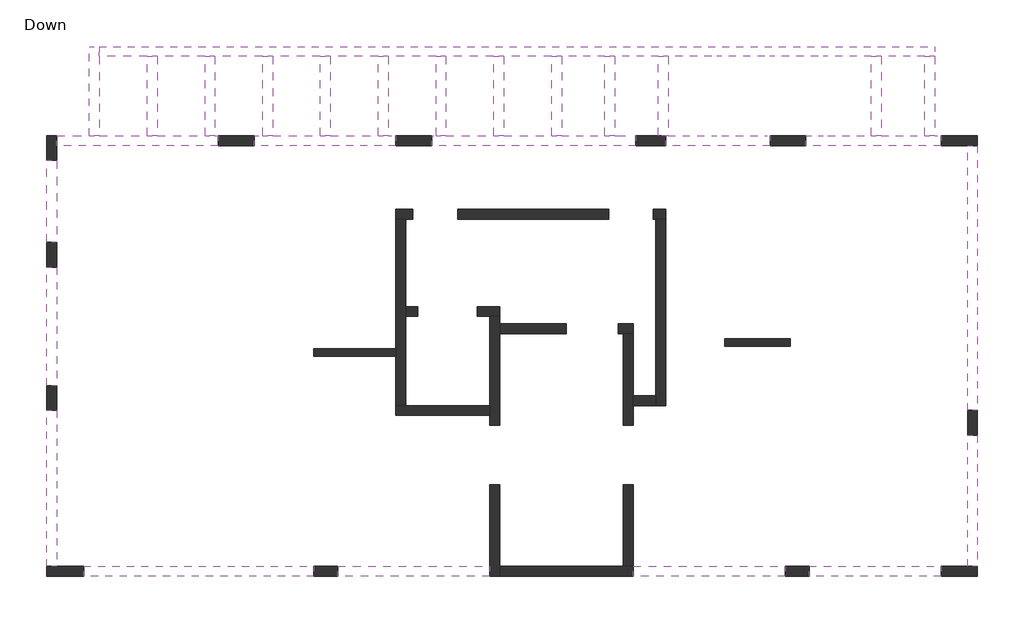
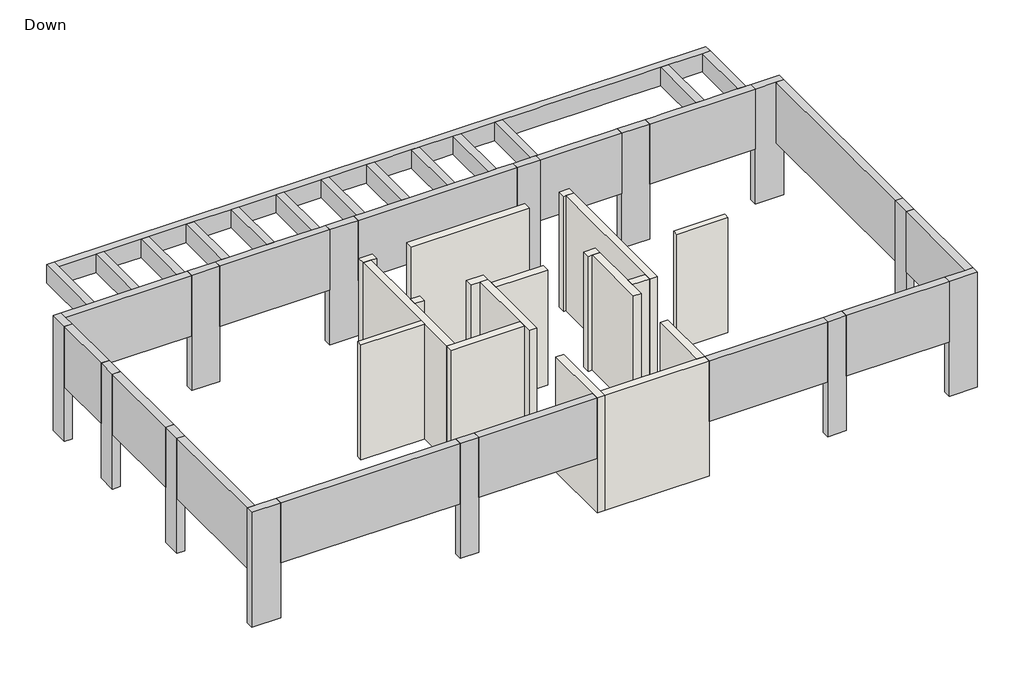
# One storey: 28 beams, 18 walls, 13 columns.
"""IFC4 building model written with IfcOpenShell, lengths in millimetres."""

from ifc_helpers import new_model, si_unit, frame, origin, origin_with_axes, place, context, project, spatial, polyline, outline, extrude, faceted_brep, element, save

model = new_model("IFC4")

# Units and contexts
model_context = context("Model", 3, world=origin())
ifc_project = project(units=[si_unit("LENGTHUNIT", "METRE", prefix="MILLI")], contexts=[model_context])

# Site, building, storey
site = spatial("IfcSite", under=ifc_project)
building = spatial("IfcBuilding", under=site)
storey = spatial("IfcBuildingStorey", under=building, Name="Down", Elevation=0.0)

# Beams
placement = place(None, origin())
element("IfcBeam", 1, ObjectType="Concrete Rectengular Beam : 20/165", at=placement, inside=storey, context=model_context, shape_type="SweptSolid", body=[
    extrude(outline(polyline([(-28799.0775982, 37234.7104697), (-28799.0775982, 37034.7104697), (-33449.2609999, 37034.7104697), (-33449.2609999, 37234.7104697), (-28799.0775982, 37234.7104697)])), frame((0.0, 0.0, 1500.0), z_axis=(0.0, 0.0, 1.0), x_axis=(1.0, 0.0, 0.0)), (0.0, 0.0, 1.0), 1650.0),
])
element("IfcBeam", 2, ObjectType="Concrete Rectengular Beam : 20/165", at=placement, inside=storey, context=model_context, shape_type="Brep", body=[
    faceted_brep([(-28319.0775982, 37234.7104697, 3150.0), (-28319.0775982, 37034.7104697, 3150.0), (-25248.1921114, 37034.7104697, 3150.0), (-25248.1921114, 37234.7104697, 3150.0), (-28319.0775982, 37034.7104697, 1500.0), (-25248.1921114, 37034.7104697, 1500.0), (-28319.0775982, 37234.7104697, 1500.0), (-25248.1921114, 37234.7104697, 1500.0), (-25248.1921114, 37234.7104697, 2950.0)], [[[0, 1, 2, 3]], [[1, 4, 5, 2]], [[4, 6, 7, 5]], [[6, 0, 3, 8, 7]], [[1, 0, 6, 4]], [[3, 2, 5, 7, 8]]]),
])
element("IfcBeam", 3, ObjectType="Concrete Rectengular Beam : 20/165", at=placement, inside=storey, context=model_context, shape_type="Brep", body=[
    faceted_brep([(-19279.0292046, 37034.7104697, 3150.0), (-19279.0292046, 37234.7104697, 3150.0), (-22348.1921114, 37234.7104697, 3150.0), (-22348.1921114, 37034.7104697, 3150.0), (-19279.0292046, 37034.7104697, 1500.0), (-22348.1921114, 37034.7104697, 1500.0), (-19279.0292046, 37234.7104697, 1500.0), (-22348.1921114, 37234.7104697, 1500.0), (-22348.1921114, 37234.7104697, 2950.0)], [[[0, 1, 2, 3]], [[4, 0, 3, 5]], [[6, 4, 5, 7]], [[1, 6, 7, 8, 2]], [[1, 0, 4, 6]], [[3, 2, 8, 7, 5]]]),
])
element("IfcBeam", 4, ObjectType="Concrete Rectengular Beam : 20/165", at=placement, inside=storey, context=model_context, shape_type="SweptSolid", body=[
    extrude(outline(polyline([(-16128.1921114, 37234.7104697), (-16128.1921114, 37034.7104697), (-18799.0292046, 37034.7104697), (-18799.0292046, 37234.7104697), (-16128.1921114, 37234.7104697)])), frame((0.0, 0.0, 1500.0), z_axis=(0.0, 0.0, 1.0), x_axis=(1.0, 0.0, 0.0)), (0.0, 0.0, 1.0), 1650.0),
])
element("IfcBeam", 5, ObjectType="Concrete Rectengular Beam : 20/165", at=placement, inside=storey, context=model_context, shape_type="Brep", body=[
    faceted_brep([(-15398.1921114, 39884.7076972, 3150.0), (-15598.1921114, 39884.7076972, 3150.0), (-15598.1921114, 37234.7104697, 3150.0), (-15398.1921114, 37234.7104697, 3150.0), (-15398.1921114, 39884.7076972, 1500.0), (-15398.1921114, 37234.7104697, 1500.0), (-15598.1921114, 39884.7076972, 1500.0), (-15598.1921114, 37234.7104697, 1500.0), (-15598.1921114, 37234.7104697, 2950.0)], [[[0, 1, 2, 3]], [[4, 0, 3, 5]], [[6, 4, 5, 7]], [[1, 6, 7, 8, 2]], [[1, 0, 4, 6]], [[3, 2, 8, 7, 5]]]),
])
element("IfcBeam", 6, ObjectType="Concrete Rectengular Beam : 20/165", at=placement, inside=storey, context=model_context, shape_type="Brep", body=[
    faceted_brep([(-15598.1921114, 40384.7076972, 3150.0), (-15398.1921114, 40384.7076972, 3150.0), (-15398.1921114, 45734.7104697, 3150.0), (-15598.1921114, 45734.7104697, 3150.0), (-15398.1921114, 40384.7076972, 1500.0), (-15398.1921114, 45734.7104697, 1500.0), (-15598.1921114, 40384.7076972, 1500.0), (-15598.1921114, 45734.7104697, 1500.0), (-15598.1921114, 45734.7104697, 2950.0)], [[[0, 1, 2, 3]], [[1, 4, 5, 2]], [[4, 6, 7, 5]], [[6, 0, 3, 8, 7]], [[1, 0, 6, 4]], [[3, 2, 5, 7, 8]]]),
])
element("IfcBeam", 7, ObjectType="Concrete Rectengular Beam : 20/165", at=placement, inside=storey, context=model_context, shape_type="Brep", body=[
    faceted_brep([(-16128.1921114, 45734.7104697, 3150.0), (-16128.1921114, 45934.7104697, 3150.0), (-16263.1921114, 45934.7104697, 3150.0), (-16463.1921114, 45934.7104697, 3150.0), (-17340.2921114, 45934.7104697, 3150.0), (-17540.2921114, 45934.7104697, 3150.0), (-18417.3921114, 45934.7104697, 3150.0), (-18617.3921114, 45934.7104697, 3150.0), (-18867.9882316, 45934.7104697, 3150.0), (-18867.9882316, 45734.7104697, 3150.0), (-16128.1921114, 45934.7104697, 1500.0), (-18867.9882316, 45934.7104697, 1500.0), (-16128.1921114, 45734.7104697, 1500.0), (-18867.9882316, 45734.7104697, 1500.0)], [[[0, 1, 2, 3, 4, 5, 6, 7, 8, 9]], [[1, 10, 11, 8, 7, 6, 5, 4, 3, 2]], [[10, 12, 13, 11]], [[12, 0, 9, 13]], [[1, 0, 12, 10]], [[9, 8, 11, 13]]]),
])
element("IfcBeam", 8, ObjectType="Concrete Rectengular Beam : 20/165", at=placement, inside=storey, context=model_context, shape_type="Brep", body=[
    faceted_brep([(-19587.9882316, 45734.7104697, 3150.0), (-19587.9882316, 45934.7104697, 3150.0), (-19694.4921114, 45934.7104697, 3150.0), (-20566.8921114, 45934.7104697, 3150.0), (-20766.8921114, 45934.7104697, 3150.0), (-21643.9921114, 45934.7104697, 3150.0), (-21697.8129925, 45934.7104697, 3150.0), (-21697.8129925, 45734.7104697, 3150.0), (-19587.9882316, 45934.7104697, 1500.0), (-21697.8129925, 45934.7104697, 1500.0), (-19587.9882316, 45734.7104697, 1500.0), (-21697.8129925, 45734.7104697, 1500.0)], [[[0, 1, 2, 3, 4, 5, 6, 7]], [[1, 8, 9, 6, 5, 4, 3, 2]], [[8, 10, 11, 9]], [[10, 0, 7, 11]], [[1, 0, 10, 8]], [[7, 6, 9, 11]]]),
])
element("IfcBeam", 9, ObjectType="Concrete Rectengular Beam : 20/165", at=placement, inside=storey, context=model_context, shape_type="Brep", body=[
    faceted_brep([(-26418.1921114, 45934.7104697, 3150.0), (-26418.1921114, 45734.7104697, 3150.0), (-22297.8129925, 45734.7104697, 3150.0), (-22297.8129925, 45934.7104697, 3150.0), (-22721.0921114, 45934.7104697, 3150.0), (-22921.0921114, 45934.7104697, 3150.0), (-23798.1921114, 45934.7104697, 3150.0), (-23998.1921114, 45934.7104697, 3150.0), (-24965.6921114, 45934.7104697, 3150.0), (-25165.6921114, 45934.7104697, 3150.0), (-26133.1921114, 45934.7104697, 3150.0), (-26333.1921114, 45934.7104697, 3150.0), (-26418.1921114, 45934.7104697, 1500.0), (-22297.8129925, 45934.7104697, 1500.0), (-26418.1921114, 45734.7104697, 1500.0), (-22297.8129925, 45734.7104697, 1500.0)], [[[0, 1, 2, 3, 4, 5, 6, 7, 8, 9, 10, 11]], [[12, 0, 11, 10, 9, 8, 7, 6, 5, 4, 3, 13]], [[14, 12, 13, 15]], [[1, 14, 15, 2]], [[1, 0, 12, 14]], [[3, 2, 15, 13]]]),
])
element("IfcBeam", 10, ObjectType="Concrete Rectengular Beam : 20/165", at=placement, inside=storey, context=model_context, shape_type="Brep", body=[
    faceted_brep([(-30003.1920714, 45934.7104697, 3150.0), (-30003.1920714, 45734.7104697, 3150.0), (-27148.1921114, 45734.7104697, 3150.0), (-27148.1921114, 45934.7104697, 3150.0), (-27300.6921114, 45934.7104697, 3150.0), (-27500.6921114, 45934.7104697, 3150.0), (-28468.1921114, 45934.7104697, 3150.0), (-28668.1921114, 45934.7104697, 3150.0), (-29630.6921114, 45934.7104697, 3150.0), (-29830.6921114, 45934.7104697, 3150.0), (-30003.1920714, 45934.7104697, 1500.0), (-27148.1921114, 45934.7104697, 1500.0), (-30003.1920714, 45734.7104697, 1500.0), (-27148.1921114, 45734.7104697, 1500.0)], [[[0, 1, 2, 3, 4, 5, 6, 7, 8, 9]], [[10, 0, 9, 8, 7, 6, 5, 4, 3, 11]], [[12, 10, 11, 13]], [[1, 12, 13, 2]], [[1, 0, 10, 12]], [[3, 2, 13, 11]]]),
])
element("IfcBeam", 11, ObjectType="Concrete Rectengular Beam : 20/165", at=placement, inside=storey, context=model_context, shape_type="Brep", body=[
    faceted_brep([(-33998.1921114, 45934.7104697, 3150.0), (-33998.1921114, 45734.7104697, 3150.0), (-30733.1920714, 45734.7104697, 3150.0), (-30733.1920714, 45934.7104697, 3150.0), (-30798.1921114, 45934.7104697, 3150.0), (-30998.1921114, 45934.7104697, 3150.0), (-31965.6921114, 45934.7104697, 3150.0), (-32165.6921114, 45934.7104697, 3150.0), (-33133.1921114, 45934.7104697, 3150.0), (-33333.1921114, 45934.7104697, 3150.0), (-33998.1921114, 45934.7104697, 1500.0), (-30733.1920714, 45934.7104697, 1500.0), (-33998.1921114, 45734.7104697, 1500.0), (-30733.1920714, 45734.7104697, 1500.0), (-33998.1921114, 45734.7104697, 2950.0)], [[[0, 1, 2, 3, 4, 5, 6, 7, 8, 9]], [[10, 0, 9, 8, 7, 6, 5, 4, 3, 11]], [[12, 10, 11, 13]], [[1, 14, 12, 13, 2]], [[1, 0, 10, 12, 14]], [[3, 2, 13, 11]]]),
])
element("IfcBeam", 12, ObjectType="Concrete Rectengular Beam : 20/165", at=placement, inside=storey, context=model_context, shape_type="SweptSolid", body=[
    extrude(outline(polyline([(-34198.1921114, 45434.7104697), (-33998.1921114, 45434.7104697), (-33998.1921114, 43778.8121651), (-34198.1921114, 43778.8121651), (-34198.1921114, 45434.7104697)])), frame((0.0, 0.0, 1500.0), z_axis=(0.0, 0.0, 1.0), x_axis=(1.0, 0.0, 0.0)), (0.0, 0.0, 1.0), 1650.0),
])
element("IfcBeam", 13, ObjectType="Concrete Rectengular Beam : 20/165", at=placement, inside=storey, context=model_context, shape_type="SweptSolid", body=[
    extrude(outline(polyline([(-34198.1921114, 43278.8121651), (-33998.1921114, 43278.8121651), (-33998.1921114, 40884.7121321), (-34198.1921114, 40884.7121321), (-34198.1921114, 43278.8121651)])), frame((0.0, 0.0, 1500.0), z_axis=(0.0, 0.0, 1.0), x_axis=(1.0, 0.0, 0.0)), (0.0, 0.0, 1.0), 1650.0),
])
element("IfcBeam", 14, ObjectType="Concrete Rectengular Beam : 20/165", at=placement, inside=storey, context=model_context, shape_type="Brep", body=[
    faceted_brep([(-33998.1921114, 40384.7121321, 3150.0), (-34198.1921114, 40384.7121321, 3150.0), (-34198.1921114, 37234.7104697, 3150.0), (-33998.1921114, 37234.7104697, 3150.0), (-34198.1921114, 40384.7121321, 1500.0), (-34198.1921114, 37234.7104697, 1500.0), (-33998.1921114, 40384.7121321, 1500.0), (-33998.1921114, 37234.7104697, 1500.0), (-33998.1921114, 37234.7104697, 2950.0)], [[[0, 1, 2, 3]], [[1, 4, 5, 2]], [[4, 6, 7, 5]], [[6, 0, 3, 8, 7]], [[1, 0, 6, 4]], [[3, 2, 5, 7, 8]]]),
])
element("IfcBeam", 15, ObjectType="Concrete Rectengular Beam : 20/50", at=placement, inside=storey, context=model_context, shape_type="Brep", body=[
    faceted_brep([(-33133.1921114, 47734.7104697, 3150.0), (-33333.1921114, 47734.7104697, 3150.0), (-33333.1921114, 45934.7104697, 3150.0), (-33133.1921114, 45934.7104697, 3150.0), (-33133.1921114, 47534.7104697, 3150.0), (-33133.1921114, 47734.7104697, 2650.0), (-33133.1921114, 45934.7104697, 2650.0), (-33133.1921114, 47534.7104697, 2650.0), (-33333.1921114, 47734.7104697, 2650.0), (-33333.1921114, 45934.7104697, 2650.0)], [[[0, 1, 2, 3, 4]], [[5, 0, 4, 3, 6, 7]], [[8, 5, 7, 6, 9]], [[1, 8, 9, 2]], [[3, 2, 9, 6]], [[1, 0, 5, 8]]]),
])
element("IfcBeam", 16, ObjectType="Concrete Rectengular Beam : 20/50", at=placement, inside=storey, context=model_context, shape_type="Brep", body=[
    faceted_brep([(-16263.1921114, 47534.7104697, 3150.0), (-16263.1921114, 47734.7104697, 3150.0), (-33133.1921114, 47734.7104697, 3150.0), (-33133.1921114, 47534.7104697, 3150.0), (-32165.6921114, 47534.7104697, 3150.0), (-31965.6921114, 47534.7104697, 3150.0), (-30998.1921114, 47534.7104697, 3150.0), (-30798.1921114, 47534.7104697, 3150.0), (-29830.6921114, 47534.7104697, 3150.0), (-29630.6921114, 47534.7104697, 3150.0), (-28668.1921114, 47534.7104697, 3150.0), (-28468.1921114, 47534.7104697, 3150.0), (-27500.6921114, 47534.7104697, 3150.0), (-27300.6921114, 47534.7104697, 3150.0), (-26333.1921114, 47534.7104697, 3150.0), (-26133.1921114, 47534.7104697, 3150.0), (-25165.6921114, 47534.7104697, 3150.0), (-24965.6921114, 47534.7104697, 3150.0), (-23998.1921114, 47534.7104697, 3150.0), (-23798.1921114, 47534.7104697, 3150.0), (-22921.0921114, 47534.7104697, 3150.0), (-22721.0921114, 47534.7104697, 3150.0), (-21843.9921114, 47534.7104697, 3150.0), (-21643.9921114, 47534.7104697, 3150.0), (-20766.8921114, 47534.7104697, 3150.0), (-20566.8921114, 47534.7104697, 3150.0), (-19694.4921114, 47534.7104697, 3150.0), (-19494.4921114, 47534.7104697, 3150.0), (-18617.3921114, 47534.7104697, 3150.0), (-18417.3921114, 47534.7104697, 3150.0), (-17540.2921114, 47534.7104697, 3150.0), (-17340.2921114, 47534.7104697, 3150.0), (-16463.1921114, 47534.7104697, 3150.0), (-16263.1921114, 47534.7104697, 2650.0), (-33133.1921114, 47534.7104697, 2650.0), (-32165.6921114, 47534.7104697, 2650.0), (-31965.6921114, 47534.7104697, 2650.0), (-30998.1921114, 47534.7104697, 2650.0), (-30798.1921114, 47534.7104697, 2650.0), (-29830.6921114, 47534.7104697, 2650.0), (-29630.6921114, 47534.7104697, 2650.0), (-28668.1921114, 47534.7104697, 2650.0), (-28468.1921114, 47534.7104697, 2650.0), (-27500.6921114, 47534.7104697, 2650.0), (-27300.6921114, 47534.7104697, 2650.0), (-26333.1921114, 47534.7104697, 2650.0), (-26133.1921114, 47534.7104697, 2650.0), (-25165.6921114, 47534.7104697, 2650.0), (-24965.6921114, 47534.7104697, 2650.0), (-23998.1921114, 47534.7104697, 2650.0), (-23798.1921114, 47534.7104697, 2650.0), (-22921.0921114, 47534.7104697, 2650.0), (-22721.0921114, 47534.7104697, 2650.0), (-21843.9921114, 47534.7104697, 2650.0), (-21643.9921114, 47534.7104697, 2650.0), (-20766.8921114, 47534.7104697, 2650.0), (-20566.8921114, 47534.7104697, 2650.0), (-19694.4921114, 47534.7104697, 2650.0), (-19494.4921114, 47534.7104697, 2650.0), (-18617.3921114, 47534.7104697, 2650.0), (-18417.3921114, 47534.7104697, 2650.0), (-17540.2921114, 47534.7104697, 2650.0), (-17340.2921114, 47534.7104697, 2650.0), (-16463.1921114, 47534.7104697, 2650.0), (-16263.1921114, 47734.7104697, 2650.0), (-33133.1921114, 47734.7104697, 2650.0)], [[[0, 1, 2, 3, 4, 5, 6, 7, 8, 9, 10, 11, 12, 13, 14, 15, 16, 17, 18, 19, 20, 21, 22, 23, 24, 25, 26, 27, 28, 29, 30, 31, 32]], [[33, 0, 32, 31, 30, 29, 28, 27, 26, 25, 24, 23, 22, 21, 20, 19, 18, 17, 16, 15, 14, 13, 12, 11, 10, 9, 8, 7, 6, 5, 4, 3, 34, 35, 36, 37, 38, 39, 40, 41, 42, 43, 44, 45, 46, 47, 48, 49, 50, 51, 52, 53, 54, 55, 56, 57, 58, 59, 60, 61, 62, 63]], [[64, 33, 63, 62, 61, 60, 59, 58, 57, 56, 55, 54, 53, 52, 51, 50, 49, 48, 47, 46, 45, 44, 43, 42, 41, 40, 39, 38, 37, 36, 35, 34, 65]], [[1, 64, 65, 2]], [[3, 2, 65, 34]], [[1, 0, 33, 64]]]),
])
element("IfcBeam", 17, ObjectType="Concrete Rectengular Beam : 20/50", at=placement, inside=storey, context=model_context, shape_type="SweptSolid", body=[
    extrude(outline(polyline([(-16463.1921114, 47534.7104697), (-16263.1921114, 47534.7104697), (-16263.1921114, 45934.7104697), (-16463.1921114, 45934.7104697), (-16463.1921114, 47534.7104697)])), frame((0.0, 0.0, 2650.0), z_axis=(0.0, 0.0, 1.0), x_axis=(1.0, 0.0, 0.0)), (0.0, 0.0, 1.0), 500.0),
])
element("IfcBeam", 18, ObjectType="Concrete Rectengular Beam : 20/50", at=placement, inside=storey, context=model_context, shape_type="SweptSolid", body=[
    extrude(outline(polyline([(-17540.2921114, 47534.7104697), (-17340.2921114, 47534.7104697), (-17340.2921114, 45934.7104697), (-17540.2921114, 45934.7104697), (-17540.2921114, 47534.7104697)])), frame((0.0, 0.0, 2650.0), z_axis=(0.0, 0.0, 1.0), x_axis=(1.0, 0.0, 0.0)), (0.0, 0.0, 1.0), 500.0),
])
element("IfcBeam", 19, ObjectType="Concrete Rectengular Beam : 20/50", at=placement, inside=storey, context=model_context, shape_type="Brep", body=[
    faceted_brep([(-21843.9921114, 45934.7104697, 3150.0), (-21697.8129925, 45934.7104697, 3150.0), (-21643.9921114, 45934.7104697, 3150.0), (-21643.9921114, 47534.7104697, 3150.0), (-21843.9921114, 47534.7104697, 3150.0), (-21843.9921114, 45934.7104697, 2650.0), (-21843.9921114, 47534.7104697, 2650.0), (-21643.9921114, 45934.7104697, 2650.0), (-21643.9921114, 47534.7104697, 2650.0)], [[[0, 1, 2, 3, 4]], [[5, 0, 4, 6]], [[7, 5, 6, 8]], [[2, 7, 8, 3]], [[2, 1, 0, 5, 7]], [[4, 3, 8, 6]]]),
])
element("IfcBeam", 20, ObjectType="Concrete Rectengular Beam : 20/50", at=placement, inside=storey, context=model_context, shape_type="SweptSolid", body=[
    extrude(outline(polyline([(-22921.0921114, 47534.7104697), (-22721.0921114, 47534.7104697), (-22721.0921114, 45934.7104697), (-22921.0921114, 45934.7104697), (-22921.0921114, 47534.7104697)])), frame((0.0, 0.0, 2650.0), z_axis=(0.0, 0.0, 1.0), x_axis=(1.0, 0.0, 0.0)), (0.0, 0.0, 1.0), 500.0),
])
element("IfcBeam", 21, ObjectType="Concrete Rectengular Beam : 20/50", at=placement, inside=storey, context=model_context, shape_type="SweptSolid", body=[
    extrude(outline(polyline([(-23798.1921114, 45934.7104697), (-23998.1921114, 45934.7104697), (-23998.1921114, 47534.7104697), (-23798.1921114, 47534.7104697), (-23798.1921114, 45934.7104697)])), frame((0.0, 0.0, 2650.0), z_axis=(0.0, 0.0, 1.0), x_axis=(1.0, 0.0, 0.0)), (0.0, 0.0, 1.0), 500.0),
])
element("IfcBeam", 22, ObjectType="Concrete Rectengular Beam : 20/50", at=placement, inside=storey, context=model_context, shape_type="SweptSolid", body=[
    extrude(outline(polyline([(-24965.6921114, 45934.7104697), (-25165.6921114, 45934.7104697), (-25165.6921114, 47534.7104697), (-24965.6921114, 47534.7104697), (-24965.6921114, 45934.7104697)])), frame((0.0, 0.0, 2650.0), z_axis=(0.0, 0.0, 1.0), x_axis=(1.0, 0.0, 0.0)), (0.0, 0.0, 1.0), 500.0),
])
element("IfcBeam", 23, ObjectType="Concrete Rectengular Beam : 20/50", at=placement, inside=storey, context=model_context, shape_type="SweptSolid", body=[
    extrude(outline(polyline([(-26133.1921114, 45934.7104697), (-26333.1921114, 45934.7104697), (-26333.1921114, 47534.7104697), (-26133.1921114, 47534.7104697), (-26133.1921114, 45934.7104697)])), frame((0.0, 0.0, 2650.0), z_axis=(0.0, 0.0, 1.0), x_axis=(1.0, 0.0, 0.0)), (0.0, 0.0, 1.0), 500.0),
])
element("IfcBeam", 24, ObjectType="Concrete Rectengular Beam : 20/50", at=placement, inside=storey, context=model_context, shape_type="SweptSolid", body=[
    extrude(outline(polyline([(-27500.6921114, 47534.7104697), (-27300.6921114, 47534.7104697), (-27300.6921114, 45934.7104697), (-27500.6921114, 45934.7104697), (-27500.6921114, 47534.7104697)])), frame((0.0, 0.0, 2650.0), z_axis=(0.0, 0.0, 1.0), x_axis=(1.0, 0.0, 0.0)), (0.0, 0.0, 1.0), 500.0),
])
element("IfcBeam", 25, ObjectType="Concrete Rectengular Beam : 20/50", at=placement, inside=storey, context=model_context, shape_type="SweptSolid", body=[
    extrude(outline(polyline([(-28468.1921114, 45934.7104697), (-28668.1921114, 45934.7104697), (-28668.1921114, 47534.7104697), (-28468.1921114, 47534.7104697), (-28468.1921114, 45934.7104697)])), frame((0.0, 0.0, 2650.0), z_axis=(0.0, 0.0, 1.0), x_axis=(1.0, 0.0, 0.0)), (0.0, 0.0, 1.0), 500.0),
])
element("IfcBeam", 26, ObjectType="Concrete Rectengular Beam : 20/50", at=placement, inside=storey, context=model_context, shape_type="SweptSolid", body=[
    extrude(outline(polyline([(-29630.6921114, 45934.7104697), (-29830.6921114, 45934.7104697), (-29830.6921114, 47534.7104697), (-29630.6921114, 47534.7104697), (-29630.6921114, 45934.7104697)])), frame((0.0, 0.0, 2650.0), z_axis=(0.0, 0.0, 1.0), x_axis=(1.0, 0.0, 0.0)), (0.0, 0.0, 1.0), 500.0),
])
element("IfcBeam", 27, ObjectType="Concrete Rectengular Beam : 20/50", at=placement, inside=storey, context=model_context, shape_type="SweptSolid", body=[
    extrude(outline(polyline([(-30798.1921114, 45934.7104697), (-30998.1921114, 45934.7104697), (-30998.1921114, 47534.7104697), (-30798.1921114, 47534.7104697), (-30798.1921114, 45934.7104697)])), frame((0.0, 0.0, 2650.0), z_axis=(0.0, 0.0, 1.0), x_axis=(1.0, 0.0, 0.0)), (0.0, 0.0, 1.0), 500.0),
])
element("IfcBeam", 28, ObjectType="Concrete Rectengular Beam : 20/50", at=placement, inside=storey, context=model_context, shape_type="SweptSolid", body=[
    extrude(outline(polyline([(-31965.6921114, 45934.7104697), (-32165.6921114, 45934.7104697), (-32165.6921114, 47534.7104697), (-31965.6921114, 47534.7104697), (-31965.6921114, 45934.7104697)])), frame((0.0, 0.0, 2650.0), z_axis=(0.0, 0.0, 1.0), x_axis=(1.0, 0.0, 0.0)), (0.0, 0.0, 1.0), 500.0),
])

# Columns
element("IfcColumn", 29, ObjectType="Concrete Rectengular Column : 20/48", at=placement, inside=storey, context=model_context, shape_type="SweptSolid", body=[
    extrude(outline(polyline([(-28799.0775982, 37234.7104697), (-28319.0775982, 37234.7104697), (-28319.0775982, 37034.7104697), (-28799.0775982, 37034.7104697), (-28799.0775982, 37234.7104697)])), origin_with_axes(), (0.0, 0.0, 1.0), 3150.0),
])
element("IfcColumn", 30, ObjectType="Concrete Rectengular Column : 20/48", at=placement, inside=storey, context=model_context, shape_type="SweptSolid", body=[
    extrude(outline(polyline([(-19279.0292046, 37234.7104697), (-18799.0292046, 37234.7104697), (-18799.0292046, 37034.7104697), (-19279.0292046, 37034.7104697), (-19279.0292046, 37234.7104697)])), origin_with_axes(), (0.0, 0.0, 1.0), 3150.0),
])
element("IfcColumn", 31, ObjectType="Concrete Rectengular Column : 20/50", at=placement, inside=storey, context=model_context, shape_type="Brep", body=[
    faceted_brep([(-33998.1921114, 45934.7104697, 0.0), (-33998.1921114, 45434.7104697, 0.0), (-34198.1921114, 45434.7104697, 0.0), (-34198.1921114, 45934.7104697, 0.0), (-33998.1921114, 45934.7104697, 3150.0), (-33998.1921114, 45734.7104697, 3150.0), (-33998.1921114, 45434.7104697, 3150.0), (-34198.1921114, 45434.7104697, 3150.0), (-34198.1921114, 45934.7104697, 3150.0)], [[[0, 1, 2, 3]], [[4, 5, 6, 1, 0]], [[6, 7, 2, 1]], [[7, 8, 3, 2]], [[8, 4, 0, 3]], [[4, 8, 7, 6, 5]]]),
])
element("IfcColumn", 32, ObjectType="Concrete Rectengular Column : 20/50", at=placement, inside=storey, context=model_context, shape_type="SweptSolid", body=[
    extrude(outline(polyline([(-33998.1921114, 43778.8121651), (-33998.1921114, 43278.8121651), (-34198.1921114, 43278.8121651), (-34198.1921114, 43778.8121651), (-33998.1921114, 43778.8121651)])), origin_with_axes(), (0.0, 0.0, 1.0), 3150.0),
])
element("IfcColumn", 33, ObjectType="Concrete Rectengular Column : 20/50", at=placement, inside=storey, context=model_context, shape_type="SweptSolid", body=[
    extrude(outline(polyline([(-33998.1921114, 40884.7121321), (-33998.1921114, 40384.7121321), (-34198.1921114, 40384.7121321), (-34198.1921114, 40884.7121321), (-33998.1921114, 40884.7121321)])), origin_with_axes(), (0.0, 0.0, 1.0), 3150.0),
])
element("IfcColumn", 34, ObjectType="Concrete Rectengular Column : 20/50", at=placement, inside=storey, context=model_context, shape_type="SweptSolid", body=[
    extrude(outline(polyline([(-15398.1921114, 40384.7076972), (-15398.1921114, 39884.7076972), (-15598.1921114, 39884.7076972), (-15598.1921114, 40384.7076972), (-15398.1921114, 40384.7076972)])), origin_with_axes(), (0.0, 0.0, 1.0), 3150.0),
])
element("IfcColumn", 35, ObjectType="Concrete Rectengular Column : 20/60", at=placement, inside=storey, context=model_context, shape_type="Brep", body=[
    faceted_brep([(-22297.8129925, 45934.7104697, 0.0), (-21697.8129925, 45934.7104697, 0.0), (-21697.8129925, 45734.7104697, 0.0), (-22297.8129925, 45734.7104697, 0.0), (-22297.8129925, 45934.7104697, 3150.0), (-21697.8129925, 45934.7104697, 3150.0), (-22297.8129925, 45934.7104697, 1500.0), (-21697.8129925, 45734.7104697, 3150.0), (-21698.192111, 45734.7104697, 3150.0), (-22297.8129925, 45734.7104697, 3150.0), (-22297.8129925, 45734.7104697, 1500.0)], [[[0, 1, 2, 3]], [[4, 5, 1, 0, 6]], [[5, 7, 2, 1]], [[7, 8, 9, 10, 3, 2]], [[9, 4, 6, 0, 3, 10]], [[4, 9, 8, 7, 5]]]),
])
element("IfcColumn", 36, ObjectType="Concrete Rectengular Column : 20/72", at=placement, inside=storey, context=model_context, shape_type="SweptSolid", body=[
    extrude(outline(polyline([(-19587.9882316, 45934.7104697), (-18867.9882316, 45934.7104697), (-18867.9882316, 45734.7104697), (-19587.9882316, 45734.7104697), (-19587.9882316, 45934.7104697)])), origin_with_axes(), (0.0, 0.0, 1.0), 3150.0),
])
element("IfcColumn", 37, ObjectType="Concrete Rectengular Column : 20/73", at=placement, inside=storey, context=model_context, shape_type="Brep", body=[
    faceted_brep([(-16128.1921114, 37234.7104697, 0.0), (-15398.1921114, 37234.7104697, 0.0), (-15398.1921114, 37034.7104697, 0.0), (-16128.1921114, 37034.7104697, 0.0), (-16128.1921114, 37234.7104697, 3150.0), (-15598.1921114, 37234.7104697, 3150.0), (-15398.1921114, 37234.7104697, 3150.0), (-15398.1921114, 37034.7104697, 3150.0), (-16128.1921114, 37034.7104697, 3150.0)], [[[0, 1, 2, 3]], [[4, 5, 6, 1, 0]], [[6, 7, 2, 1]], [[7, 8, 3, 2]], [[8, 4, 0, 3]], [[4, 8, 7, 6, 5]]]),
])
element("IfcColumn", 38, ObjectType="Concrete Rectengular Column : 20/73", at=placement, inside=storey, context=model_context, shape_type="Brep", body=[
    faceted_brep([(-16128.1921114, 45934.7104697, 0.0), (-15398.1921114, 45934.7104697, 0.0), (-15398.1921114, 45734.7104697, 0.0), (-16128.1921114, 45734.7104697, 0.0), (-16128.1921114, 45934.7104697, 3150.0), (-15398.1921114, 45934.7104697, 3150.0), (-15398.1921114, 45734.7104697, 3150.0), (-15598.1921114, 45734.7104697, 3150.0), (-16128.1921114, 45734.7104697, 3150.0)], [[[0, 1, 2, 3]], [[4, 5, 1, 0]], [[5, 6, 2, 1]], [[6, 7, 8, 3, 2]], [[8, 4, 0, 3]], [[4, 8, 7, 6, 5]]]),
])
element("IfcColumn", 39, ObjectType="Concrete Rectengular Column : 20/73", at=placement, inside=storey, context=model_context, shape_type="SweptSolid", body=[
    extrude(outline(polyline([(-30733.1920714, 45934.7104697), (-30003.1920714, 45934.7104697), (-30003.1920714, 45734.7104697), (-30733.1920714, 45734.7104697), (-30733.1920714, 45934.7104697)])), origin_with_axes(), (0.0, 0.0, 1.0), 3150.0),
])
element("IfcColumn", 40, ObjectType="Concrete Rectengular Column : 20/73", at=placement, inside=storey, context=model_context, shape_type="SweptSolid", body=[
    extrude(outline(polyline([(-27148.1921114, 45934.7104697), (-26418.1921114, 45934.7104697), (-26418.1921114, 45734.7104697), (-27148.1921114, 45734.7104697), (-27148.1921114, 45934.7104697)])), origin_with_axes(), (0.0, 0.0, 1.0), 3150.0),
])
element("IfcColumn", 41, ObjectType="Concrete Rectengular Column : 20/75", at=placement, inside=storey, context=model_context, shape_type="Brep", body=[
    faceted_brep([(-34199.2609999, 37234.7104697, 0.0), (-33449.2609999, 37234.7104697, 0.0), (-33449.2609999, 37034.7104697, 0.0), (-34199.2609999, 37034.7104697, 0.0), (-34199.2609999, 37234.7104697, 3150.0), (-33998.1921114, 37234.7104697, 3150.0), (-33449.2609999, 37234.7104697, 3150.0), (-33449.2609999, 37034.7104697, 3150.0), (-34199.2609999, 37034.7104697, 3150.0)], [[[0, 1, 2, 3]], [[4, 5, 6, 1, 0]], [[6, 7, 2, 1]], [[7, 8, 3, 2]], [[8, 4, 0, 3]], [[4, 8, 7, 6, 5]]]),
])

# Walls
element("IfcWall", 42, ObjectType="15", at=placement, inside=storey, context=model_context, shape_type="Brep", body=[
    faceted_brep([(-28798.1921114, 41484.7104697, 0.0), (-27148.1921114, 41484.7104697, 0.0), (-27148.1921114, 41484.7104697, 2950.0), (-27148.1921114, 41484.7104697, 3150.0), (-28798.1921114, 41484.7104697, 3150.0), (-28798.1921114, 41484.7104697, 2950.0), (-28798.1921114, 41634.7104697, 0.0), (-28798.1921114, 41634.7104697, 2950.0), (-28798.1921114, 41634.7104697, 3150.0), (-27148.1921114, 41634.7104697, 3150.0), (-27148.1921114, 41634.7104697, 2950.0), (-27148.1921114, 41634.7104697, 0.0)], [[[0, 1, 2, 3, 4, 5]], [[6, 7, 8, 9, 10, 11]], [[1, 0, 6, 11]], [[4, 3, 9, 8]], [[0, 5, 4, 8, 7, 6]], [[3, 2, 1, 11, 10, 9]]]),
])
element("IfcWall", 43, ObjectType="15", at=placement, inside=storey, context=model_context, shape_type="Brep", body=[
    faceted_brep([(-19178.1921114, 41834.7104349, 0.0), (-20498.1921114, 41834.7104349, 0.0), (-20498.1921114, 41834.7104349, 2950.0), (-20498.1921114, 41834.7104349, 3150.0), (-19178.1921114, 41834.7104349, 3150.0), (-19178.1921114, 41834.7104349, 2950.0), (-19178.1921114, 41684.7104349, 0.0), (-19178.1921114, 41684.7104349, 2950.0), (-19178.1921114, 41684.7104349, 3150.0), (-20498.1921114, 41684.7104349, 3150.0), (-20498.1921114, 41684.7104349, 2950.0), (-20498.1921114, 41684.7104349, 0.0)], [[[0, 1, 2, 3, 4, 5]], [[6, 7, 8, 9, 10, 11]], [[1, 0, 6, 11]], [[3, 2, 1, 11, 10, 9]], [[4, 3, 9, 8]], [[0, 5, 4, 8, 7, 6]]]),
])
element("IfcWall", 44, ObjectType="20", at=placement, inside=storey, context=model_context, shape_type="Brep", body=[
    faceted_brep([(-25248.1921114, 38884.7104697, 0.0), (-25248.1921114, 37034.7104697, 0.0), (-25248.1921114, 37034.7104697, 3150.0), (-25248.1921114, 37234.7104697, 3150.0), (-25248.1921114, 38884.7104697, 3150.0), (-25248.1921114, 38884.7104697, 2950.0), (-25048.1921114, 38884.7104697, 0.0), (-25048.1921114, 38884.7104697, 2950.0), (-25048.1921114, 38884.7104697, 3150.0), (-25048.1921114, 37234.7104697, 3150.0), (-25048.1921114, 37034.7104697, 3150.0), (-25048.1921114, 37034.7104697, 0.0), (-25048.1921114, 37234.7104697, 0.0)], [[[0, 1, 2, 3, 4, 5]], [[6, 7, 8, 9, 10, 11, 12]], [[1, 0, 6, 12, 11]], [[4, 3, 2, 10, 9, 8]], [[0, 5, 4, 8, 7, 6]], [[2, 1, 11, 10]]]),
])
element("IfcWall", 45, ObjectType="20", at=placement, inside=storey, context=model_context, shape_type="Brep", body=[
    faceted_brep([(-25048.1921114, 37034.7104697, 0.0), (-22348.1921114, 37034.7104697, 0.0), (-22348.1921114, 37034.7104697, 1500.0), (-22348.1921114, 37034.7104697, 3150.0), (-25048.1921114, 37034.7104697, 3150.0), (-25048.1921114, 37234.7104697, 0.0), (-25048.1921114, 37234.7104697, 3150.0), (-22548.1921114, 37234.7104697, 3150.0), (-22348.1921114, 37234.7104697, 3150.0), (-22348.1921114, 37234.7104697, 1500.0), (-22348.1921114, 37234.7104697, 0.0), (-22548.1921114, 37234.7104697, 0.0)], [[[0, 1, 2, 3, 4]], [[5, 6, 7, 8, 9, 10, 11]], [[1, 0, 5, 11, 10]], [[4, 3, 8, 7, 6]], [[0, 4, 6, 5]], [[3, 2, 1, 10, 9, 8]]]),
])
element("IfcWall", 46, ObjectType="20", at=placement, inside=storey, context=model_context, shape_type="Brep", body=[
    faceted_brep([(-22348.1921114, 37234.7104697, 0.0), (-22348.1921114, 38884.7104697, 0.0), (-22348.1921114, 38884.7104697, 2950.0), (-22348.1921114, 38884.7104697, 3150.0), (-22348.1921114, 37234.7104697, 3150.0), (-22348.1921114, 37234.7104697, 2950.0), (-22548.1921114, 37234.7104697, 0.0), (-22548.1921114, 37234.7104697, 3150.0), (-22548.1921114, 38884.7104697, 3150.0), (-22548.1921114, 38884.7104697, 2950.0), (-22548.1921114, 38884.7104697, 0.0)], [[[0, 1, 2, 3, 4, 5]], [[6, 7, 8, 9, 10]], [[1, 0, 6, 10]], [[3, 2, 1, 10, 9, 8]], [[4, 3, 8, 7]], [[0, 5, 4, 7, 6]]]),
])
element("IfcWall", 47, ObjectType="20", at=placement, inside=storey, context=model_context, shape_type="Brep", body=[
    faceted_brep([(-22348.1921114, 40084.7104697, 0.0), (-22348.1921114, 40484.7104697, 0.0), (-22348.1921114, 40684.7104697, 0.0), (-22348.1921114, 41934.7104698, 0.0), (-22348.1921114, 41934.7104698, 3150.0), (-22348.1921114, 40684.7104697, 3150.0), (-22348.1921114, 40484.7104697, 3150.0), (-22348.1921114, 40084.7104697, 3150.0), (-22348.1921114, 40084.7104697, 2950.0), (-22548.1921114, 40084.7104697, 0.0), (-22548.1921114, 40084.7104697, 2950.0), (-22548.1921114, 40084.7104697, 3150.0), (-22548.1921114, 41934.7104698, 3150.0), (-22548.1921114, 41934.7104698, 0.0)], [[[0, 1, 2, 3, 4, 5, 6, 7, 8]], [[9, 10, 11, 12, 13]], [[3, 2, 1, 0, 9, 13]], [[7, 6, 5, 4, 12, 11]], [[0, 8, 7, 11, 10, 9]], [[4, 3, 13, 12]]]),
])
element("IfcWall", 48, ObjectType="20", at=placement, inside=storey, context=model_context, shape_type="Brep", body=[
    faceted_brep([(-22348.1921114, 42134.7104698, 0.0), (-22648.1921114, 42134.7104698, 0.0), (-22648.1921114, 42134.7104698, 2950.0), (-22648.1921114, 42134.7104698, 3150.0), (-22348.1921114, 42134.7104698, 3150.0), (-22348.1921114, 42134.7104698, 2950.0), (-22348.1921114, 41934.7104698, 0.0), (-22348.1921114, 41934.7104698, 3150.0), (-22548.1921114, 41934.7104698, 3150.0), (-22648.1921114, 41934.7104698, 3150.0), (-22648.1921114, 41934.7104698, 2950.0), (-22648.1921114, 41934.7104698, 0.0), (-22548.1921114, 41934.7104698, 0.0)], [[[0, 1, 2, 3, 4, 5]], [[6, 7, 8, 9, 10, 11, 12]], [[1, 0, 6, 12, 11]], [[3, 2, 1, 11, 10, 9]], [[4, 3, 9, 8, 7]], [[0, 5, 4, 7, 6]]]),
])
element("IfcWall", 49, ObjectType="20", at=placement, inside=storey, context=model_context, shape_type="Brep", body=[
    faceted_brep([(-23698.1921114, 42134.7104697, 0.0), (-25048.1921114, 42134.7104697, 0.0), (-25048.1921114, 42134.7104697, 2950.0), (-25048.1921114, 42134.7104697, 3150.0), (-23698.1921114, 42134.7104697, 3150.0), (-23698.1921114, 42134.7104697, 2950.0), (-23698.1921114, 41934.7104697, 0.0), (-23698.1921114, 41934.7104697, 2950.0), (-23698.1921114, 41934.7104697, 3150.0), (-25048.1921114, 41934.7104697, 3150.0), (-25048.1921114, 41934.7104697, 0.0)], [[[0, 1, 2, 3, 4, 5]], [[6, 7, 8, 9, 10]], [[1, 0, 6, 10]], [[4, 3, 9, 8]], [[0, 5, 4, 8, 7, 6]], [[3, 2, 1, 10, 9]]]),
])
element("IfcWall", 50, ObjectType="20", at=placement, inside=storey, context=model_context, shape_type="Brep", body=[
    faceted_brep([(-25248.1921114, 42284.7104696, 0.0), (-25248.1921114, 40484.7104697, 0.0), (-25248.1921114, 40284.7104697, 0.0), (-25248.1921114, 40084.7104697, 0.0), (-25248.1921114, 40084.7104697, 2950.0), (-25248.1921114, 40084.7104697, 3150.0), (-25248.1921114, 40284.7104697, 3150.0), (-25248.1921114, 40484.7104697, 3150.0), (-25248.1921114, 42284.7104696, 3150.0), (-25248.1921114, 42284.7104696, 2950.0), (-25048.1921114, 42284.7104696, 0.0), (-25048.1921114, 42284.7104696, 3150.0), (-25048.1921114, 42134.7104697, 3150.0), (-25048.1921114, 41934.7104697, 3150.0), (-25048.1921114, 40084.7104697, 3150.0), (-25048.1921114, 40084.7104697, 2950.0), (-25048.1921114, 40084.7104697, 0.0), (-25048.1921114, 41934.7104697, 0.0), (-25048.1921114, 42134.7104697, 0.0)], [[[0, 1, 2, 3, 4, 5, 6, 7, 8, 9]], [[10, 11, 12, 13, 14, 15, 16, 17, 18]], [[3, 2, 1, 0, 10, 18, 17, 16]], [[5, 4, 3, 16, 15, 14]], [[8, 7, 6, 5, 14, 13, 12, 11]], [[0, 9, 8, 11, 10]]]),
])
element("IfcWall", 51, ObjectType="20", at=placement, inside=storey, context=model_context, shape_type="Brep", body=[
    faceted_brep([(-25248.1921114, 40484.7104697, 0.0), (-26948.1921114, 40484.7104697, 0.0), (-27148.1921114, 40484.7104697, 0.0), (-27148.1921114, 40484.7104697, 3150.0), (-26948.1921114, 40484.7104697, 3150.0), (-25248.1921114, 40484.7104697, 3150.0), (-25248.1921114, 40484.7104697, 2950.0), (-25248.1921114, 40284.7104697, 0.0), (-25248.1921114, 40284.7104697, 2950.0), (-25248.1921114, 40284.7104697, 3150.0), (-27148.1921114, 40284.7104697, 3150.0), (-27148.1921114, 40284.7104697, 2950.0), (-27148.1921114, 40284.7104697, 0.0)], [[[0, 1, 2, 3, 4, 5, 6]], [[7, 8, 9, 10, 11, 12]], [[2, 1, 0, 7, 12]], [[5, 4, 3, 10, 9]], [[0, 6, 5, 9, 8, 7]], [[3, 2, 12, 11, 10]]]),
])
element("IfcWall", 52, ObjectType="20", at=placement, inside=storey, context=model_context, shape_type="Brep", body=[
    faceted_brep([(-26948.1921114, 40484.7104697, 0.0), (-26948.1921114, 42284.7104697, 0.0), (-26948.1921114, 42484.7104697, 0.0), (-26948.1921114, 44244.7104697, 0.0), (-26948.1921114, 44244.7104697, 2950.0), (-26948.1921114, 44244.7104697, 3150.0), (-26948.1921114, 42484.7104697, 3150.0), (-26948.1921114, 42284.7104697, 3150.0), (-26948.1921114, 40484.7104697, 3150.0), (-26948.1921114, 40484.7104697, 2950.0), (-27148.1921114, 40484.7104697, 0.0), (-27148.1921114, 40484.7104697, 3150.0), (-27148.1921114, 41484.7104697, 3150.0), (-27148.1921114, 41634.7104697, 3150.0), (-27148.1921114, 44244.7104697, 3150.0), (-27148.1921114, 44244.7104697, 0.0), (-27148.1921114, 41634.7104697, 0.0), (-27148.1921114, 41484.7104697, 0.0)], [[[0, 1, 2, 3, 4, 5, 6, 7, 8, 9]], [[10, 11, 12, 13, 14, 15, 16, 17]], [[3, 2, 1, 0, 10, 17, 16, 15]], [[8, 7, 6, 5, 14, 13, 12, 11]], [[0, 9, 8, 11, 10]], [[5, 4, 3, 15, 14]]]),
])
element("IfcWall", 53, ObjectType="20", at=placement, inside=storey, context=model_context, shape_type="Brep", body=[
    faceted_brep([(-27148.1921114, 44244.7104697, 0.0), (-26948.1921114, 44244.7104697, 0.0), (-26798.1921114, 44244.7104697, 0.0), (-26798.1921114, 44244.7104697, 2950.0), (-26798.1921114, 44244.7104697, 3150.0), (-26948.1921114, 44244.7104697, 3150.0), (-27148.1921114, 44244.7104697, 3150.0), (-27148.1921114, 44444.7104697, 0.0), (-27148.1921114, 44444.7104697, 2950.0), (-27148.1921114, 44444.7104697, 3150.0), (-26798.1921114, 44444.7104697, 3150.0), (-26798.1921114, 44444.7104697, 2950.0), (-26798.1921114, 44444.7104697, 0.0)], [[[0, 1, 2, 3, 4, 5, 6]], [[7, 8, 9, 10, 11, 12]], [[2, 1, 0, 7, 12]], [[4, 3, 2, 12, 11, 10]], [[6, 5, 4, 10, 9]], [[0, 6, 9, 8, 7]]]),
])
element("IfcWall", 54, ObjectType="20", at=placement, inside=storey, context=model_context, shape_type="Brep", body=[
    faceted_brep([(-25898.1921114, 44244.7104697, 0.0), (-22848.1921114, 44244.7104697, 0.0), (-22848.1921114, 44244.7104697, 2950.0), (-22848.1921114, 44244.7104697, 3150.0), (-25898.1921114, 44244.7104697, 3150.0), (-25898.1921114, 44244.7104697, 2950.0), (-25898.1921114, 44444.7104697, 0.0), (-25898.1921114, 44444.7104697, 2950.0), (-25898.1921114, 44444.7104697, 3150.0), (-22848.1921114, 44444.7104697, 3150.0), (-22848.1921114, 44444.7104697, 2950.0), (-22848.1921114, 44444.7104697, 0.0)], [[[0, 1, 2, 3, 4, 5]], [[6, 7, 8, 9, 10, 11]], [[1, 0, 6, 11]], [[3, 2, 1, 11, 10, 9]], [[4, 3, 9, 8]], [[0, 5, 4, 8, 7, 6]]]),
])
element("IfcWall", 55, ObjectType="20", at=placement, inside=storey, context=model_context, shape_type="Brep", body=[
    faceted_brep([(-21948.1921114, 44244.7104697, 0.0), (-21898.192111, 44244.7104697, 0.0), (-21698.192111, 44244.7104697, 0.0), (-21698.192111, 44244.7104697, 3150.0), (-21898.192111, 44244.7104697, 3150.0), (-21948.1921114, 44244.7104697, 3150.0), (-21948.1921114, 44244.7104697, 2950.0), (-21948.1921114, 44444.7104697, 0.0), (-21948.1921114, 44444.7104697, 2950.0), (-21948.1921114, 44444.7104697, 3150.0), (-21698.192111, 44444.7104697, 3150.0), (-21698.192111, 44444.7104697, 2950.0), (-21698.192111, 44444.7104697, 0.0)], [[[0, 1, 2, 3, 4, 5, 6]], [[7, 8, 9, 10, 11, 12]], [[2, 1, 0, 7, 12]], [[5, 4, 3, 10, 9]], [[0, 6, 5, 9, 8, 7]], [[3, 2, 12, 11, 10]]]),
])
element("IfcWall", 56, ObjectType="20", at=placement, inside=storey, context=model_context, shape_type="Brep", body=[
    faceted_brep([(-21898.192111, 44244.7104697, 0.0), (-21898.192111, 40684.7104697, 0.0), (-21898.192111, 40484.7104697, 0.0), (-21898.192111, 40484.7104697, 3150.0), (-21898.192111, 40684.7104697, 3150.0), (-21898.192111, 44244.7104697, 3150.0), (-21898.192111, 44244.7104697, 2950.0), (-21698.192111, 44244.7104697, 0.0), (-21698.192111, 44244.7104697, 3150.0), (-21698.192111, 40484.7104697, 3150.0), (-21698.192111, 40484.7104697, 2950.0), (-21698.192111, 40484.7104697, 0.0)], [[[0, 1, 2, 3, 4, 5, 6]], [[7, 8, 9, 10, 11]], [[2, 1, 0, 7, 11]], [[5, 4, 3, 9, 8]], [[0, 6, 5, 8, 7]], [[3, 2, 11, 10, 9]]]),
])
element("IfcWall", 57, ObjectType="20", at=placement, inside=storey, context=model_context, shape_type="Brep", body=[
    faceted_brep([(-21898.192111, 40684.7104697, 0.0), (-22348.1921114, 40684.7104697, 0.0), (-22348.1921114, 40684.7104697, 2950.0), (-22348.1921114, 40684.7104697, 3150.0), (-21898.192111, 40684.7104697, 3150.0), (-21898.192111, 40684.7104697, 2950.0), (-21898.192111, 40484.7104697, 0.0), (-21898.192111, 40484.7104697, 3150.0), (-22348.1921114, 40484.7104697, 3150.0), (-22348.1921114, 40484.7104697, 2950.0), (-22348.1921114, 40484.7104697, 0.0)], [[[0, 1, 2, 3, 4, 5]], [[6, 7, 8, 9, 10]], [[1, 0, 6, 10]], [[4, 3, 8, 7]], [[0, 5, 4, 7, 6]], [[3, 2, 1, 10, 9, 8]]]),
])
element("IfcWall", 58, ObjectType="20", at=placement, inside=storey, context=model_context, shape_type="Brep", body=[
    faceted_brep([(-25048.1921114, 42484.7104696, 0.0), (-25498.1921114, 42484.7104696, 0.0), (-25498.1921114, 42484.7104696, 2950.0), (-25498.1921114, 42484.7104696, 3150.0), (-25048.1921114, 42484.7104696, 3150.0), (-25048.1921114, 42484.7104696, 2950.0), (-25048.1921114, 42284.7104696, 0.0), (-25048.1921114, 42284.7104696, 3150.0), (-25248.1921114, 42284.7104696, 3150.0), (-25498.1921114, 42284.7104696, 3150.0), (-25498.1921114, 42284.7104696, 2950.0), (-25498.1921114, 42284.7104696, 0.0), (-25248.1921114, 42284.7104696, 0.0)], [[[0, 1, 2, 3, 4, 5]], [[6, 7, 8, 9, 10, 11, 12]], [[1, 0, 6, 12, 11]], [[3, 2, 1, 11, 10, 9]], [[4, 3, 9, 8, 7]], [[0, 5, 4, 7, 6]]]),
])
element("IfcWall", 59, ObjectType="20", at=placement, inside=storey, context=model_context, shape_type="Brep", body=[
    faceted_brep([(-26698.1921114, 42484.7104697, 0.0), (-26948.1921114, 42484.7104697, 0.0), (-26948.1921114, 42484.7104697, 2950.0), (-26948.1921114, 42484.7104697, 3150.0), (-26698.1921114, 42484.7104697, 3150.0), (-26698.1921114, 42484.7104697, 2950.0), (-26698.1921114, 42284.7104697, 0.0), (-26698.1921114, 42284.7104697, 2950.0), (-26698.1921114, 42284.7104697, 3150.0), (-26948.1921114, 42284.7104697, 3150.0), (-26948.1921114, 42284.7104697, 2950.0), (-26948.1921114, 42284.7104697, 0.0)], [[[0, 1, 2, 3, 4, 5]], [[6, 7, 8, 9, 10, 11]], [[1, 0, 6, 11]], [[4, 3, 9, 8]], [[0, 5, 4, 8, 7, 6]], [[3, 2, 1, 11, 10, 9]]]),
])

save(model, "model.ifc")

# Revit data of these elements
# Project information
#   Project Issue Date = "Issue Date"
#   Project Status = "Project Status"
#   Client Name = "לקוח"
#   Project Address = "Enter address here"
#   Project Name = "Project 047"
#   Project Number = "מספר פרויקט"
# Type "Concrete Rectengular Beam : 20/165"
#   Length [instance default] = 152.4 cm
#   b = 20 cm
#   h = 165 cm
#   Structural Material [instance default] = Concrete
#   Assembly Code = ""
# Type "Concrete Rectengular Beam : 20/50"
#   Length [instance default] = 152.4 cm
#   b = 20 cm
#   h = 50 cm
#   Structural Material [instance default] = Concrete
#   Assembly Code = ""
# Type "Concrete Rectengular Column : 20/48"
#   b = 20 cm
#   h = 48 cm
#   Structural Material [instance default] = Concrete
# Type "Concrete Rectengular Column : 20/50"
#   b = 20 cm
#   h = 50 cm
#   Structural Material [instance default] = Concrete
# Type "Concrete Rectengular Column : 20/60"
#   b = 20 cm
#   h = 60 cm
#   Structural Material [instance default] = Concrete
# Type "Concrete Rectengular Column : 20/72"
#   b = 20 cm
#   h = 72 cm
#   Structural Material [instance default] = Concrete
# Type "Concrete Rectengular Column : 20/73"
#   b = 20 cm
#   h = 73 cm
#   Structural Material [instance default] = Concrete
# Type "Concrete Rectengular Column : 20/75"
#   b = 20 cm
#   h = 75 cm
#   Structural Material [instance default] = Concrete
# Type "15"
#   Layers, outside or top first: 15 cm "Concrete" (function 1)
# Type "20"
#   Layers, outside or top first: 20 cm "Concrete" (function 1)
# Element 1 (IfcBeam, "Concrete Rectengular Beam : 20/165")
#   Comments = ""
#   Mark = "B1"
#   SOFiSTiK_AMG_Comments = ""
#   SOFiSTiK_AMG_Scheduled = yes
#   SOFiSTiK_AMG_Adjusted = yes
#   Structural Material = Concrete
#   Phase Created = New Construction
#   Materials on its faces: "Concrete"
# Element 2 (IfcBeam, "Concrete Rectengular Beam : 20/165")
#   Comments = ""
#   Mark = "B2"
#   SOFiSTiK_AMG_Comments = ""
#   SOFiSTiK_AMG_Scheduled = yes
#   SOFiSTiK_AMG_Adjusted = yes
#   Structural Material = Concrete
#   Phase Created = New Construction
#   Materials on its faces: "Concrete"
# Element 3 (IfcBeam, "Concrete Rectengular Beam : 20/165")
#   Comments = ""
#   Mark = "B3"
#   SOFiSTiK_AMG_Comments = ""
#   SOFiSTiK_AMG_Scheduled = yes
#   SOFiSTiK_AMG_Adjusted = yes
#   Structural Material = Concrete
#   Phase Created = New Construction
#   Materials on its faces: "Concrete"
# Element 4 (IfcBeam, "Concrete Rectengular Beam : 20/165")
#   Comments = ""
#   Mark = "B4"
#   SOFiSTiK_AMG_Comments = ""
#   SOFiSTiK_AMG_Scheduled = yes
#   SOFiSTiK_AMG_Adjusted = yes
#   Structural Material = Concrete
#   Phase Created = New Construction
#   Materials on its faces: "Concrete"
# Element 5 (IfcBeam, "Concrete Rectengular Beam : 20/165")
#   Comments = ""
#   Mark = "B5"
#   SOFiSTiK_AMG_Comments = ""
#   SOFiSTiK_AMG_Scheduled = yes
#   SOFiSTiK_AMG_Adjusted = yes
#   Structural Material = Concrete
#   Phase Created = New Construction
#   Materials on its faces: "Concrete"
# Element 6 (IfcBeam, "Concrete Rectengular Beam : 20/165")
#   Comments = ""
#   Mark = "B6"
#   SOFiSTiK_AMG_Comments = ""
#   SOFiSTiK_AMG_Scheduled = yes
#   SOFiSTiK_AMG_Adjusted = yes
#   Structural Material = Concrete
#   Phase Created = New Construction
#   Materials on its faces: "Concrete"
# Element 7 (IfcBeam, "Concrete Rectengular Beam : 20/165")
#   Comments = ""
#   Mark = "B7"
#   SOFiSTiK_AMG_Comments = ""
#   SOFiSTiK_AMG_Scheduled = yes
#   SOFiSTiK_AMG_Adjusted = yes
#   Structural Material = Concrete
#   Phase Created = New Construction
#   Materials on its faces: "Concrete"
# Element 8 (IfcBeam, "Concrete Rectengular Beam : 20/165")
#   Comments = ""
#   Mark = "B8"
#   SOFiSTiK_AMG_Comments = ""
#   SOFiSTiK_AMG_Scheduled = yes
#   SOFiSTiK_AMG_Adjusted = yes
#   Structural Material = Concrete
#   Phase Created = New Construction
#   Materials on its faces: "Concrete"
# Element 9 (IfcBeam, "Concrete Rectengular Beam : 20/165")
#   Comments = ""
#   Mark = "B9"
#   SOFiSTiK_AMG_Comments = ""
#   SOFiSTiK_AMG_Scheduled = yes
#   SOFiSTiK_AMG_Adjusted = yes
#   Structural Material = Concrete
#   Phase Created = New Construction
#   Materials on its faces: "Concrete"
# Element 10 (IfcBeam, "Concrete Rectengular Beam : 20/165")
#   Comments = ""
#   Mark = "B10"
#   SOFiSTiK_AMG_Comments = ""
#   SOFiSTiK_AMG_Scheduled = yes
#   SOFiSTiK_AMG_Adjusted = yes
#   Structural Material = Concrete
#   Phase Created = New Construction
#   Materials on its faces: "Concrete"
# Element 11 (IfcBeam, "Concrete Rectengular Beam : 20/165")
#   Comments = ""
#   Mark = "B11"
#   SOFiSTiK_AMG_Comments = ""
#   SOFiSTiK_AMG_Scheduled = yes
#   SOFiSTiK_AMG_Adjusted = yes
#   Structural Material = Concrete
#   Phase Created = New Construction
#   Materials on its faces: "Concrete"
# Element 12 (IfcBeam, "Concrete Rectengular Beam : 20/165")
#   Comments = ""
#   Mark = "B12"
#   SOFiSTiK_AMG_Comments = ""
#   SOFiSTiK_AMG_Scheduled = yes
#   SOFiSTiK_AMG_Adjusted = yes
#   Structural Material = Concrete
#   Phase Created = New Construction
#   Materials on its faces: "Concrete"
# Element 13 (IfcBeam, "Concrete Rectengular Beam : 20/165")
#   Comments = ""
#   Mark = "B13"
#   SOFiSTiK_AMG_Comments = ""
#   SOFiSTiK_AMG_Scheduled = yes
#   SOFiSTiK_AMG_Adjusted = yes
#   Structural Material = Concrete
#   Phase Created = New Construction
#   Materials on its faces: "Concrete"
# Element 14 (IfcBeam, "Concrete Rectengular Beam : 20/165")
#   Comments = ""
#   Mark = "B14"
#   SOFiSTiK_AMG_Comments = ""
#   SOFiSTiK_AMG_Scheduled = yes
#   SOFiSTiK_AMG_Adjusted = yes
#   Structural Material = Concrete
#   Phase Created = New Construction
#   Materials on its faces: "Concrete"
# Element 15 (IfcBeam, "Concrete Rectengular Beam : 20/50")
#   Comments = ""
#   Mark = "B15"
#   SOFiSTiK_AMG_Comments = ""
#   SOFiSTiK_AMG_Scheduled = yes
#   SOFiSTiK_AMG_Adjusted = yes
#   Structural Material = Concrete
#   Phase Created = New Construction
#   Materials on its faces: "Concrete"
# Element 16 (IfcBeam, "Concrete Rectengular Beam : 20/50")
#   Comments = ""
#   Mark = "B16"
#   SOFiSTiK_AMG_Comments = ""
#   SOFiSTiK_AMG_Scheduled = yes
#   SOFiSTiK_AMG_Adjusted = yes
#   Structural Material = Concrete
#   Phase Created = New Construction
#   Materials on its faces: "Concrete"
# Element 17 (IfcBeam, "Concrete Rectengular Beam : 20/50")
#   Comments = ""
#   Mark = "B17"
#   SOFiSTiK_AMG_Comments = ""
#   SOFiSTiK_AMG_Scheduled = yes
#   SOFiSTiK_AMG_Adjusted = yes
#   Structural Material = Concrete
#   Phase Created = New Construction
#   Materials on its faces: "Concrete"
# Element 18 (IfcBeam, "Concrete Rectengular Beam : 20/50")
#   Comments = ""
#   Mark = "B18"
#   SOFiSTiK_AMG_Comments = ""
#   SOFiSTiK_AMG_Scheduled = yes
#   SOFiSTiK_AMG_Adjusted = yes
#   Structural Material = Concrete
#   Phase Created = New Construction
#   Materials on its faces: "Concrete"
# Element 19 (IfcBeam, "Concrete Rectengular Beam : 20/50")
#   Comments = ""
#   Mark = "B22"
#   SOFiSTiK_AMG_Comments = ""
#   SOFiSTiK_AMG_Scheduled = yes
#   SOFiSTiK_AMG_Adjusted = yes
#   Structural Material = Concrete
#   Phase Created = New Construction
#   Materials on its faces: "Concrete"
# Element 20 (IfcBeam, "Concrete Rectengular Beam : 20/50")
#   Comments = ""
#   Mark = "B23"
#   SOFiSTiK_AMG_Comments = ""
#   SOFiSTiK_AMG_Scheduled = yes
#   SOFiSTiK_AMG_Adjusted = yes
#   Structural Material = Concrete
#   Phase Created = New Construction
#   Materials on its faces: "Concrete"
# Element 21 (IfcBeam, "Concrete Rectengular Beam : 20/50")
#   Comments = ""
#   Mark = "B24"
#   SOFiSTiK_AMG_Comments = ""
#   SOFiSTiK_AMG_Scheduled = yes
#   SOFiSTiK_AMG_Adjusted = yes
#   Structural Material = Concrete
#   Phase Created = New Construction
#   Materials on its faces: "Concrete"
# Element 22 (IfcBeam, "Concrete Rectengular Beam : 20/50")
#   Comments = ""
#   Mark = "B25"
#   SOFiSTiK_AMG_Comments = ""
#   SOFiSTiK_AMG_Scheduled = yes
#   SOFiSTiK_AMG_Adjusted = yes
#   Structural Material = Concrete
#   Phase Created = New Construction
#   Materials on its faces: "Concrete"
# Element 23 (IfcBeam, "Concrete Rectengular Beam : 20/50")
#   Comments = ""
#   Mark = "B26"
#   SOFiSTiK_AMG_Comments = ""
#   SOFiSTiK_AMG_Scheduled = yes
#   SOFiSTiK_AMG_Adjusted = yes
#   Structural Material = Concrete
#   Phase Created = New Construction
#   Materials on its faces: "Concrete"
# Element 24 (IfcBeam, "Concrete Rectengular Beam : 20/50")
#   Comments = ""
#   Mark = "B27"
#   SOFiSTiK_AMG_Comments = ""
#   SOFiSTiK_AMG_Scheduled = yes
#   SOFiSTiK_AMG_Adjusted = yes
#   Structural Material = Concrete
#   Phase Created = New Construction
#   Materials on its faces: "Concrete"
# Element 25 (IfcBeam, "Concrete Rectengular Beam : 20/50")
#   Comments = ""
#   Mark = "B28"
#   SOFiSTiK_AMG_Comments = ""
#   SOFiSTiK_AMG_Scheduled = yes
#   SOFiSTiK_AMG_Adjusted = yes
#   Structural Material = Concrete
#   Phase Created = New Construction
#   Materials on its faces: "Concrete"
# Element 26 (IfcBeam, "Concrete Rectengular Beam : 20/50")
#   Comments = ""
#   Mark = "B29"
#   SOFiSTiK_AMG_Comments = ""
#   SOFiSTiK_AMG_Scheduled = yes
#   SOFiSTiK_AMG_Adjusted = yes
#   Structural Material = Concrete
#   Phase Created = New Construction
#   Materials on its faces: "Concrete"
# Element 27 (IfcBeam, "Concrete Rectengular Beam : 20/50")
#   Comments = ""
#   Mark = "B30"
#   SOFiSTiK_AMG_Comments = ""
#   SOFiSTiK_AMG_Scheduled = yes
#   SOFiSTiK_AMG_Adjusted = yes
#   Structural Material = Concrete
#   Phase Created = New Construction
#   Materials on its faces: "Concrete"
# Element 28 (IfcBeam, "Concrete Rectengular Beam : 20/50")
#   Comments = ""
#   Mark = "B31"
#   SOFiSTiK_AMG_Comments = ""
#   SOFiSTiK_AMG_Scheduled = yes
#   SOFiSTiK_AMG_Adjusted = yes
#   Structural Material = Concrete
#   Phase Created = New Construction
#   Materials on its faces: "Concrete"
# Element 29 (IfcColumn, "Concrete Rectengular Column : 20/48")
#   Comments = ""
#   Mark = "C1"
#   SOFiSTiK_AMG_Comments = ""
#   SOFiSTiK_AMG_Scheduled = yes
#   SOFiSTiK_AMG_Adjusted = yes
#   Structural Material = Concrete
#   Phase Created = New Construction
#   Materials on its faces: "Concrete"
# Element 30 (IfcColumn, "Concrete Rectengular Column : 20/48")
#   Comments = ""
#   Mark = "C2"
#   SOFiSTiK_AMG_Comments = ""
#   SOFiSTiK_AMG_Scheduled = yes
#   SOFiSTiK_AMG_Adjusted = yes
#   Structural Material = Concrete
#   Phase Created = New Construction
#   Materials on its faces: "Concrete"
# Element 31 (IfcColumn, "Concrete Rectengular Column : 20/50")
#   Comments = ""
#   Mark = "C3"
#   SOFiSTiK_AMG_Comments = ""
#   SOFiSTiK_AMG_Scheduled = yes
#   SOFiSTiK_AMG_Adjusted = yes
#   Structural Material = Concrete
#   Phase Created = New Construction
#   Materials on its faces: "Concrete"
# Element 32 (IfcColumn, "Concrete Rectengular Column : 20/50")
#   Comments = ""
#   Mark = "C4"
#   SOFiSTiK_AMG_Comments = ""
#   SOFiSTiK_AMG_Scheduled = yes
#   SOFiSTiK_AMG_Adjusted = yes
#   Structural Material = Concrete
#   Phase Created = New Construction
#   Materials on its faces: "Concrete"
# Element 33 (IfcColumn, "Concrete Rectengular Column : 20/50")
#   Comments = ""
#   Mark = "C5"
#   SOFiSTiK_AMG_Comments = ""
#   SOFiSTiK_AMG_Scheduled = yes
#   SOFiSTiK_AMG_Adjusted = yes
#   Structural Material = Concrete
#   Phase Created = New Construction
#   Materials on its faces: "Concrete"
# Element 34 (IfcColumn, "Concrete Rectengular Column : 20/50")
#   Comments = ""
#   Mark = "C6"
#   SOFiSTiK_AMG_Comments = ""
#   SOFiSTiK_AMG_Scheduled = yes
#   SOFiSTiK_AMG_Adjusted = yes
#   Structural Material = Concrete
#   Phase Created = New Construction
#   Materials on its faces: "Concrete"
# Element 35 (IfcColumn, "Concrete Rectengular Column : 20/60")
#   Comments = ""
